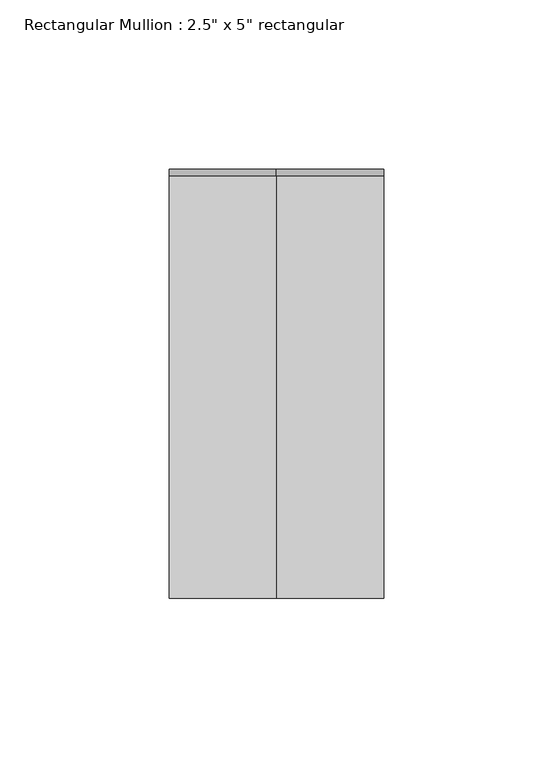
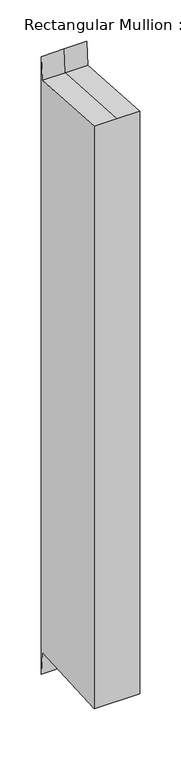
"""IFC4 building model written with IfcOpenShell, lengths in millimetres: member geometry."""

from ifc_helpers import new_model, si_unit, origin, place, context, project, spatial, faceted_brep, source, transform, mapped, element, save


def member_7c546d85(model_context):
    return source(origin(), model_context, "Body", "Brep", [
        faceted_brep([(-31.75, 63.5, 29.7846233), (0.0, 63.5, 29.7846233), (31.75, 63.5, 29.7846233), (31.75, 63.5, -880.6846233), (-31.75, 63.5, -880.6846233), (-31.75, -63.5, 3.8736342), (-31.75, 61.4149606, -3.8662198), (-31.75, 61.4149606, -847.0337802), (-31.75, -63.5, -854.7736342), (31.75, -63.5, 3.8736342), (0.0, -63.5, 3.8736342), (31.75, -63.5, -854.7736342), (31.75, 61.4149606, -3.8662198), (31.75, 61.4149606, -847.0337802), (0.0, 61.4149606, -3.8662198)], [[[0, 1, 2, 3, 4]], [[5, 6, 0, 4, 7, 8]], [[9, 10, 5, 8, 11]], [[2, 12, 9, 11, 13, 3]], [[2, 1, 14, 12]], [[1, 0, 6, 14]], [[6, 5, 10, 14]], [[10, 9, 12, 14]], [[3, 13, 7, 4]], [[13, 11, 8, 7]]]),
    ])


if __name__ == "__main__":
    model = new_model("IFC4")
    model_context = context("Model", 3, world=origin())
    ifc_project = project(units=[si_unit("LENGTHUNIT", "METRE", prefix="MILLI")], contexts=[model_context])
    site = spatial("IfcSite", under=ifc_project)
    building = spatial("IfcBuilding", under=site)
    placement = place(None, origin())
    member_shape = member_7c546d85(model_context)
    element("IfcMember", 1, ObjectType="Rectangular Mullion : 2.5\" x 5\" rectangular", at=placement, inside=building, context=model_context, shape_type="MappedRepresentation", body=[
        mapped(member_shape, transform((0.0, 0.0, 0.0), x_axis=(1.0, 0.0, 0.0), y_axis=(0.0, 1.0, 0.0), z_axis=(0.0, 0.0, 1.0))),
    ])
    save(model, "model.ifc")

# Revit data of these elements
# Type "Rectangular Mullion : 2.5\" x 5\" rectangular"
#   built-in parameter 1007304 = 0.416667 (stored number, unit not read)
#   built-in parameter 1007301 = 0.104167 (stored number, unit not read)
#   built-in parameter 1007300 = 0.104167 (stored number, unit not read)
# Element 1 (IfcMember, "Rectangular Mullion : 2.5\" x 5\" rectangular")
#   Materials on its faces: "Metal - Aluminum"
# Materials
#   "Metal - Aluminum": class "Metal", colour RGB 247 247 247, transparency 0, Cost = 0
